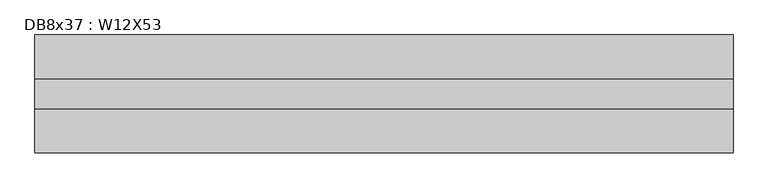
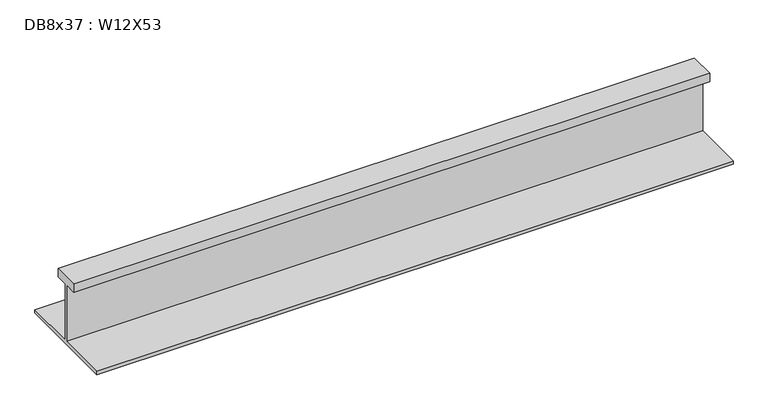
"""IFC4 building model written with IfcOpenShell, lengths in millimetres: beam geometry, DB8x37 : W12X53."""

from ifc_helpers import new_model, si_unit, frame, origin, place, context, project, spatial, polyline, outline, extrude, source, transform, mapped, element, save


def db8x37_w12x53_300c3b95(model_context):
    return source(origin(), model_context, "Body", "SweptSolid", [
        extrude(outline(polyline([(38.1, 145.415), (38.1, 120.015), (2.921, 120.015), (2.921, -48.4505), (152.4, -48.4505), (152.4, -58.1025), (-152.4, -58.1025), (-152.4, -48.4505), (-2.921, -48.4505), (-2.921, 120.015), (-38.1, 120.015), (-38.1, 145.415), (38.1, 145.415)])), frame((-851.408, 0.0, 0.0), z_axis=(1.0, 0.0, 0.0), x_axis=(0.0, 1.0, 0.0)), (0.0, 0.0, 1.0), 1803.9079994),
    ])


if __name__ == "__main__":
    model = new_model("IFC4")
    model_context = context("Model", 3, world=origin())
    ifc_project = project(units=[si_unit("LENGTHUNIT", "METRE", prefix="MILLI")], contexts=[model_context])
    site = spatial("IfcSite", under=ifc_project)
    building = spatial("IfcBuilding", under=site)
    placement = place(None, origin())
    db8x37_w12x53_shape = db8x37_w12x53_300c3b95(model_context)
    element("IfcBeam", 1, ObjectType="DB8x37 : W12X53", at=placement, inside=building, context=model_context, shape_type="MappedRepresentation", body=[
        mapped(db8x37_w12x53_shape, transform((0.0, 0.0, 0.0), x_axis=(1.0, 0.0, 0.0), y_axis=(0.0, 1.0, 0.0), z_axis=(0.0, 0.0, 1.0))),
    ])
    save(model, "model.ifc")

# Revit data of these elements
# Type "DB8x37 : W12X53"
#   Assembly Code = "B10"
#   W = 53
#   Length [instance default] = 5' - 0"
#   bf = 0' - 10"
#   d = 1' - 0.1"
#   k = 0' - 1 3/8"
#   k2 = 0' - 0.8"
#   tf = 0' - 0.575"
#   tw = 0' - 0.345"
#   A = 0.108333 SF
#   Structural Material [instance default] = Steel ASTM A992
# Element 1 (IfcBeam, "DB8x37 : W12X53")
#   Materials on its faces: "Steel ASTM A992"
# Materials
#   "Steel ASTM A992": class "Metal", colour RGB 199 199 199, transparency 0, Description = "Structural steel 50ksi", Cost = 0
